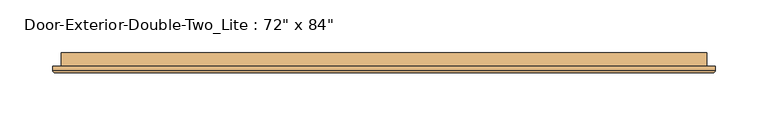
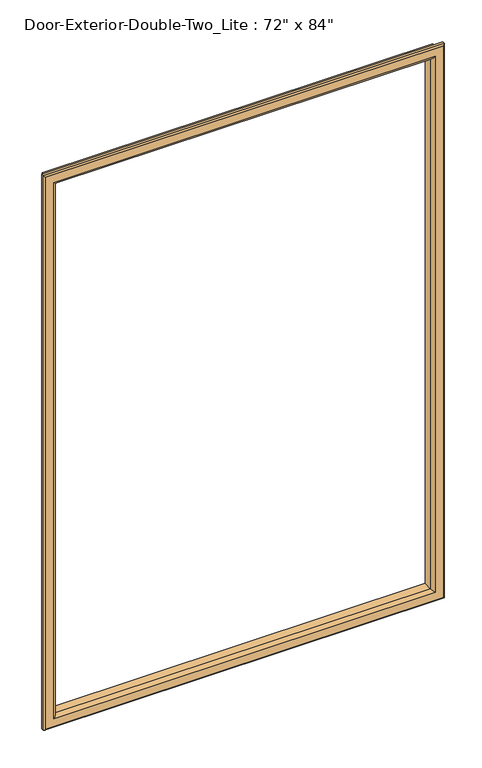
"""IFC4 building model written with IfcOpenShell, lengths in millimetres: door geometry."""

from ifc_helpers import new_model, si_unit, frame, origin, place, context, project, spatial, ellipse_curve, source, transform, mapped, element, save
from ifc_brep_helpers import plane_surface, cylinder_surface, advanced_brep


def door_d7bfd8b5(model_context):
    return source(origin(), model_context, "Body", "AdvancedBrep", [
        advanced_brep(
        [(-762.0, 52.3875, 1117.6), (-762.0, 39.6875, 1117.6), (-762.0, 39.6875, 2016.125), (-762.0, 52.3875, 2016.125), (-750.0, 38.6875, 1129.6), (-750.0, 52.3875, 1129.6), (-750.0, 52.3875, 2004.125), (-750.0, 38.6875, 2004.125), (-755.0, 33.6875, 1124.6), (-755.0, 33.6875, 2009.125), (-770.0, 35.6875, 1109.6), (-768.0, 33.6875, 1111.6), (-768.0, 33.6875, 2022.125), (-770.0, 35.6875, 2024.125), (-770.0, 39.6875, 1109.6), (-770.0, 39.6875, 2024.125), (-152.4, 39.6875, 2016.125), (-152.4, 52.3875, 2016.125), (-164.4, 52.3875, 2004.125), (-164.4, 38.6875, 2004.125), (-159.4, 33.6875, 2009.125), (-146.4, 33.6875, 2022.125), (-144.4, 35.6875, 2024.125), (-144.4, 39.6875, 2024.125), (-152.4, 39.6875, 1117.6), (-152.4, 52.3875, 1117.6), (-164.4, 52.3875, 1129.6), (-164.4, 38.6875, 1129.6), (-159.4, 33.6875, 1124.6), (-146.4, 33.6875, 1111.6), (-144.4, 35.6875, 1109.6), (-144.4, 39.6875, 1109.6)],
        [
            (0, 1),
            (1, 2),
            (2, 3),
            (3, 0),
            (4, 5),
            (5, 6),
            (6, 7),
            (7, 4),
            (8, 4, ellipse_curve(frame((-755.0, 38.6875, 1124.6), z_axis=(-0.7071067811865475, 0.0, 0.7071067811865475), x_axis=(-0.7071067811865474, 0.0, -0.7071067811865476)), 7.0710678, 5.0)),
            (7, 9, ellipse_curve(frame((-755.0, 38.6875, 2009.125), z_axis=(-0.7071067811865475, 0.0, -0.7071067811865475), x_axis=(0.7071067811865474, 0.0, -0.7071067811865476)), 7.0710678, 5.0)),
            (9, 8),
            (10, 11, ellipse_curve(frame((-768.0, 35.6875, 1111.6), z_axis=(-0.7071067811865475, 0.0, 0.7071067811865475), x_axis=(-0.7071067811865474, 0.0, -0.7071067811865476)), 2.8284271, 2.0)),
            (11, 12),
            (12, 13, ellipse_curve(frame((-768.0, 35.6875, 2022.125), z_axis=(-0.7071067811865475, 0.0, -0.7071067811865475), x_axis=(0.7071067811865474, 0.0, -0.7071067811865476)), 2.8284271, 2.0)),
            (13, 10),
            (14, 10),
            (13, 15),
            (15, 14),
            (2, 16),
            (16, 17),
            (17, 3),
            (6, 18),
            (18, 19),
            (19, 7),
            (19, 20, ellipse_curve(frame((-159.4, 38.6875, 2009.125), z_axis=(-0.7071067811865475, 0.0, 0.7071067811865475), x_axis=(-0.7071067811865476, 0.0, -0.7071067811865474)), 7.0710678, 5.0)),
            (20, 9),
            (12, 21),
            (21, 22, ellipse_curve(frame((-146.4, 35.6875, 2022.125), z_axis=(-0.7071067811865475, 0.0, 0.7071067811865475), x_axis=(-0.7071067811865476, 0.0, -0.7071067811865474)), 2.8284271, 2.0)),
            (22, 13),
            (22, 23),
            (23, 15),
            (16, 24),
            (24, 25),
            (25, 17),
            (18, 26),
            (26, 27),
            (27, 19),
            (27, 28, ellipse_curve(frame((-159.4, 38.6875, 1124.6), z_axis=(0.7071067811865475, 0.0, 0.7071067811865475), x_axis=(-0.7071067811865474, 0.0, 0.7071067811865476)), 7.0710678, 5.0)),
            (28, 20),
            (21, 29),
            (29, 30, ellipse_curve(frame((-146.4, 35.6875, 1111.6), z_axis=(0.7071067811865475, 0.0, 0.7071067811865475), x_axis=(-0.7071067811865474, 0.0, 0.7071067811865476)), 2.8284271, 2.0)),
            (30, 22),
            (30, 31),
            (31, 23),
            (31, 14),
            (1, 24),
            (0, 25),
            (5, 26),
            (4, 27),
            (8, 28),
            (11, 29),
            (10, 30),
        ],
        [
            plane_surface(frame((-762.0, 39.6875, 1117.6), z_axis=(-1.0, 0.0, 0.0), x_axis=(0.0, 0.0, 1.0))),
            plane_surface(frame((-750.0, 52.3875, 1129.6), z_axis=(1.0, 0.0, 0.0), x_axis=(0.0, 0.0, 1.0))),
            cylinder_surface(frame((-755.0, 38.6875, 1117.6), z_axis=(0.0, 0.0, -1.0), x_axis=(-1.0, 0.0, 0.0)), 5.0),
            cylinder_surface(frame((-768.0, 35.6875, 1117.6), z_axis=(0.0, 0.0, -1.0), x_axis=(-1.0, 0.0, 0.0)), 2.0),
            plane_surface(frame((-770.0, 35.6875, 1109.6), z_axis=(-1.0, 0.0, 0.0), x_axis=(0.0, 0.0, 1.0))),
            plane_surface(frame((-762.0, 39.6875, 2016.125), z_axis=(0.0, 0.0, 1.0), x_axis=(1.0, 0.0, 0.0))),
            plane_surface(frame((-750.0, 52.3875, 2004.125), z_axis=(0.0, 0.0, -1.0), x_axis=(1.0, 0.0, 0.0))),
            cylinder_surface(frame((-762.0, 38.6875, 2009.125), z_axis=(-1.0, 0.0, 0.0), x_axis=(0.0, 0.0, 1.0)), 5.0),
            cylinder_surface(frame((-762.0, 35.6875, 2022.125), z_axis=(-1.0, 0.0, 0.0), x_axis=(0.0, 0.0, 1.0)), 2.0),
            plane_surface(frame((-770.0, 35.6875, 2024.125), z_axis=(0.0, 0.0, 1.0), x_axis=(1.0, 0.0, 0.0))),
            plane_surface(frame((-152.4, 39.6875, 2016.125), z_axis=(1.0, 0.0, 0.0), x_axis=(0.0, 0.0, -1.0))),
            plane_surface(frame((-164.4, 52.3875, 2004.125), z_axis=(-1.0, 0.0, 0.0), x_axis=(0.0, 0.0, -1.0))),
            cylinder_surface(frame((-159.4, 38.6875, 2016.125), z_axis=(0.0, 0.0, 1.0), x_axis=(1.0, 0.0, 0.0)), 5.0),
            cylinder_surface(frame((-146.4, 35.6875, 2016.125), z_axis=(0.0, 0.0, 1.0), x_axis=(1.0, 0.0, 0.0)), 2.0),
            plane_surface(frame((-144.4, 35.6875, 2024.125), z_axis=(1.0, 0.0, 0.0), x_axis=(0.0, 0.0, -1.0))),
            plane_surface(frame((-144.4, 39.6875, 1109.6), z_axis=(0.0, 1.0, 0.0), x_axis=(-1.0, 0.0, 0.0))),
            plane_surface(frame((-152.4, 39.6875, 1117.6), z_axis=(0.0, 0.0, -1.0), x_axis=(-1.0, 0.0, 0.0))),
            plane_surface(frame((-152.4, 52.3875, 1117.6), z_axis=(0.0, 1.0, 0.0), x_axis=(-1.0, 0.0, 0.0))),
            plane_surface(frame((-164.4, 52.3875, 1129.6), z_axis=(0.0, 0.0, 1.0), x_axis=(-1.0, 0.0, 0.0))),
            cylinder_surface(frame((-152.4, 38.6875, 1124.6), z_axis=(1.0, 0.0, 0.0), x_axis=(0.0, 0.0, -1.0)), 5.0),
            plane_surface(frame((-159.4, 33.6875, 1124.6), z_axis=(0.0, -1.0, 0.0), x_axis=(-1.0, 0.0, 0.0))),
            cylinder_surface(frame((-152.4, 35.6875, 1111.6), z_axis=(1.0, 0.0, 0.0), x_axis=(0.0, 0.0, -1.0)), 2.0),
            plane_surface(frame((-144.4, 35.6875, 1109.6), z_axis=(0.0, 0.0, -1.0), x_axis=(-1.0, 0.0, 0.0))),
        ],
        [
            (0, [[1, 2, 3, 4]]),
            (1, [[5, 6, 7, 8]]),
            (2, [[9, -8, 10, 11]]),
            (3, [[12, 13, 14, 15]]),
            (4, [[16, -15, 17, 18]]),
            (5, [[-3, 19, 20, 21]]),
            (6, [[-7, 22, 23, 24]]),
            (7, [[-10, -24, 25, 26]]),
            (8, [[-14, 27, 28, 29]]),
            (9, [[-17, -29, 30, 31]]),
            (10, [[-20, 32, 33, 34]]),
            (11, [[-23, 35, 36, 37]]),
            (12, [[-25, -37, 38, 39]]),
            (13, [[-28, 40, 41, 42]]),
            (14, [[-30, -42, 43, 44]]),
            (15, [[-31, -44, 45, -18], [46, -32, -19, -2]]),
            (16, [[-33, -46, -1, 47]]),
            (17, [[-21, -34, -47, -4], [48, -35, -22, -6]]),
            (18, [[-36, -48, -5, 49]]),
            (19, [[-38, -49, -9, 50]]),
            (20, [[51, -40, -27, -13], [-26, -39, -50, -11]]),
            (21, [[-41, -51, -12, 52]]),
            (22, [[-43, -52, -16, -45]]),
        ],
    ),
    ])


if __name__ == "__main__":
    model = new_model("IFC4")
    model_context = context("Model", 3, world=origin())
    ifc_project = project(units=[si_unit("LENGTHUNIT", "METRE", prefix="MILLI")], contexts=[model_context])
    site = spatial("IfcSite", under=ifc_project)
    building = spatial("IfcBuilding", under=site)
    placement = place(None, origin())
    door_shape = door_d7bfd8b5(model_context)
    element("IfcDoor", 1, ObjectType="Door-Exterior-Double-Two_Lite : 72\" x 84\"", at=placement, inside=building, context=model_context, shape_type="MappedRepresentation", body=[
        mapped(door_shape, transform((0.0, 0.0, 0.0), x_axis=(1.0, 0.0, 0.0), y_axis=(0.0, 1.0, 0.0), z_axis=(0.0, 0.0, 1.0))),
    ])
    save(model, "model.ifc")

# Revit data of these elements
# Type "Door-Exterior-Double-Two_Lite : 72\" x 84\""
#   Type Mark = "20"
#   Assembly Code = "B2030100"
#   Analytic Construction = "Metal frame, double glass door"
#   Top Rail = 0' - 4 5/8"
#   Threshold Length [instance default] = 6' - 4"
#   Threshold Offset [instance default] = 0' - 0 1/2"
#   Thickness = 0' - 1 3/4"
#   Thermal Resistance (R) = 1.3794 (h·ft²·°F)/BTU
#   Swing Angle [instance default] = 90.00°
#   Strike Height = 3' - 4"
#   Stiles = 0' - 6"
#   SinglePanelWidth = 3' - 0"
#   Rough Width [instance default] = 6' - 4"
#   Rough Height [instance default] = 7' - 4"
#   MFOpeningHeight [instance default] = 0' - 4"
#   MFOpeningWidth [instance default] = 0' - 4"
#   Lock Rail = 0' - 8"
#   Inset Calculate [instance default] = 0' - 4"
#   Masonry Inset [instance default] = 0' - 1"
#   Height = 7' - 0"
#   Width = 6' - 0"
#   Heat Transfer Coefficient (U) = 0.7250 BTU/(h·ft²·°F)
#   Glass Thickness = 0' - 0 3/4"
#   Masonry Frame Depth = 0' - 5 3/4"
#   Bottom Rail = 0' - 10"
#   Threshold [instance default] = yes
#   Masonry Frame [instance default] = yes
#   Function = 1
#   Dry Wall Frame [instance default] = no
#   Threshold Material = none
#   Panic Bar Material = Metal - Stainless Steel
#   Panel Material = Metal - Painted - Grey
#   Glass Stop Material = Metal - Painted - Grey
#   Frame Material = Metal - Painted - Grey
#   Exterior Pull Material = Metal - Stainless Steel
#   Visual Light Transmittance = 0
#   Solar Heat Gain Coefficient = 0
#   Wall Closure = (empty or 0)
# Element 1 (IfcDoor, "Door-Exterior-Double-Two_Lite : 72\" x 84\"")
#   Threshold Length = 6' - 0"
#   Rough Width = 6' - 2 1/2"
#   Rough Height = 7' - 1 1/4"
#   MFOpeningHeight = 0' - 1 1/4"
#   MFOpeningWidth = 0' - 2 1/2"
#   Inset Calculate = 0' - 3"
#   Masonry Frame = no
#   Dry Wall Frame = yes
#   Materials on its faces: "Metal - Painted - Grey", "Metal - Stainless Steel", "Glass"
# Materials
#   "Metal - Stainless Steel": class "Metal", colour RGB 247 247 247, transparency 0
#   "Metal - Painted - Grey": class "Paint", colour RGB 104 104 104, transparency 0, Cost = 0
#   "Glass": class "Glass", colour RGB 0 128 192, transparency 0.75, Description = "Soda Lime Glass", Cost = 0
